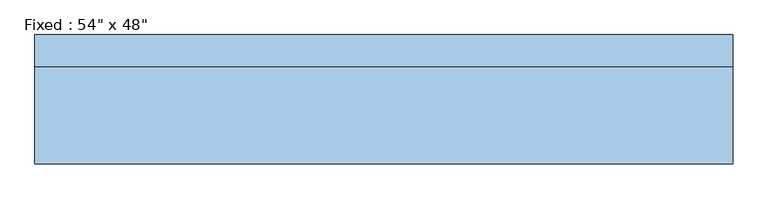
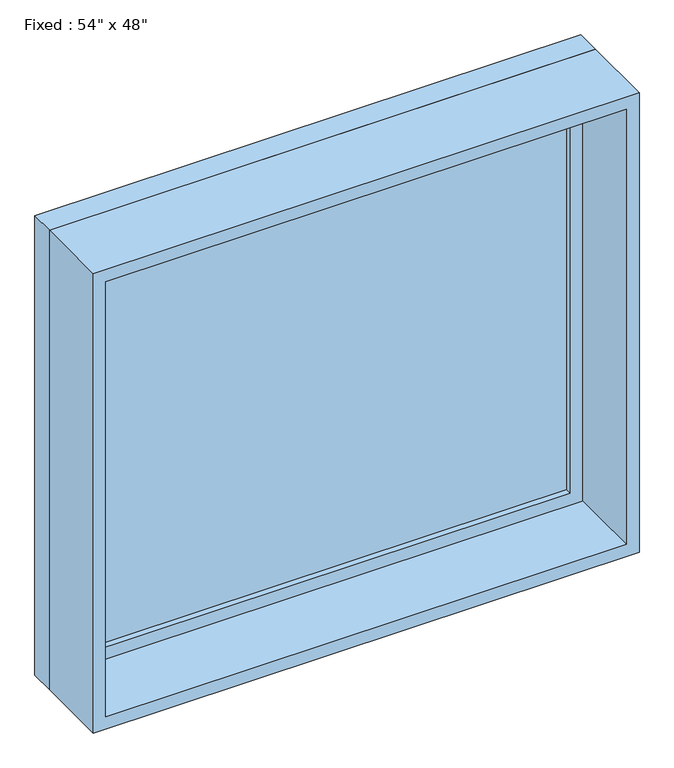
"""IFC4 building model written with IfcOpenShell, lengths in millimetres: window geometry."""

import ifcopenshell
import ifcopenshell.guid

model = None  # the IFC model being written
_history = None  # IfcOwnerHistory: only IFC2X3 demands one
_inside = {}  # id of a spatial element -> (the spatial element, [elements in it])
_under = {}  # id of a project, library or spatial element -> (it, [spatial elements below it])
_declared = {}  # id of a project -> (the project, [libraries it declares])
_typed = {}  # id of a type object -> (the type object, [elements of that type])
_made_of = {}  # id of a material, layer set ... -> (it, [elements and type objects made of it])


def new_model(schema):
    """Start an empty IFC model of exactly this schema.

    Asked for "IFC4X3", IfcOpenShell would pick the latest addendum, in which some entities
    have other attributes; the version numbers below select the first issue.
    IFC2X3 requires an IfcOwnerHistory on every rooted entity: one is made here for all.
    """
    global model, _history
    if schema == "IFC4X3":
        model = ifcopenshell.file(schema_version=(4, 3, 0, 0))
    else:
        model = ifcopenshell.file(schema=schema)
    _inside.clear()
    _under.clear()
    _declared.clear()
    _typed.clear()
    _made_of.clear()
    _history = None
    if model.schema == "IFC2X3":
        org = make("IfcOrganization", Name="unknown")
        user = make(
            "IfcPersonAndOrganization",
            ThePerson=make("IfcPerson", FamilyName="unknown"),
            TheOrganization=org,
        )
        app = make(
            "IfcApplication",
            ApplicationDeveloper=org,
            Version="unknown",
            ApplicationFullName="unknown",
            ApplicationIdentifier="unknown",
        )
        _history = make(
            "IfcOwnerHistory",
            OwningUser=user,
            OwningApplication=app,
            ChangeAction="ADDED",
            CreationDate=0,
        )
    return model


def make(cls, **values):
    """One entity of the class cls with the attributes given. An attribute that is None is left unset."""
    return model.create_entity(
        cls, **{name: value for name, value in values.items() if value is not None}
    )


def rooted(cls, **values):
    """An entity with a GlobalId (a new one), such as an element, a storey or a relation."""
    return make(cls, GlobalId=ifcopenshell.guid.new(), OwnerHistory=_history, **values)


def si_unit(unit_type, name, prefix=None):
    """IfcSIUnit, for example si_unit("LENGTHUNIT", "METRE", prefix="MILLI")."""
    return make("IfcSIUnit", UnitType=unit_type, Prefix=prefix, Name=name)


def assignment(units):
    """IfcUnitAssignment: the units of a project."""
    return None if units is None else make("IfcUnitAssignment", Units=units)


def point(xyz):
    """IfcCartesianPoint."""
    return None if xyz is None else make("IfcCartesianPoint", Coordinates=xyz)


def direction(xyz):
    """IfcDirection."""
    return None if xyz is None else make("IfcDirection", DirectionRatios=xyz)


def frame(location, z_axis=None, x_axis=None):
    """IfcAxis2Placement3D, a coordinate frame: its origin and axes. An axis left out is left unset."""
    return make(
        "IfcAxis2Placement3D",
        Location=point(location),
        Axis=direction(z_axis),
        RefDirection=direction(x_axis),
    )


def origin():
    """The frame at (0, 0, 0) with its axes left unset."""
    return frame((0.0, 0.0, 0.0))


def place(relative_to, where):
    """IfcLocalPlacement: puts the frame where relative to a parent placement (None: the world)."""
    return make(
        "IfcLocalPlacement", PlacementRelTo=relative_to, RelativePlacement=where
    )


def context(
    kind, dimensions, precision=None, world=None, true_north=None, identifier=None
):
    """IfcGeometricRepresentationContext, for example the 3D "Model" context."""
    return make(
        "IfcGeometricRepresentationContext",
        ContextIdentifier=identifier,
        ContextType=kind,
        CoordinateSpaceDimension=dimensions,
        Precision=precision,
        WorldCoordinateSystem=world,
        TrueNorth=true_north,
    )


def project(units=None, contexts=None):
    """IfcProject with its units and contexts."""
    return rooted(
        "IfcProject",
        Name="project",
        RepresentationContexts=contexts,
        UnitsInContext=assignment(units),
    )


def spatial(cls, under=None, at=None, **own):
    """A site, building, storey or space (cls), placed at a placement, below another one or the project."""
    s = rooted(cls, ObjectPlacement=at, **own)
    if under is not None:
        _under.setdefault(under.id(), (under, []))[1].append(s)
    return s


def polyline(points):
    """IfcPolyline through the points."""
    return make("IfcPolyline", Points=[point(p) for p in points])


def outline(outer, holes=None, kind="AREA"):
    """IfcArbitraryClosedProfileDef: a profile drawn as a closed curve; with holes, ...WithVoids."""
    if holes is None:
        return make("IfcArbitraryClosedProfileDef", ProfileType=kind, OuterCurve=outer)
    return make(
        "IfcArbitraryProfileDefWithVoids",
        ProfileType=kind,
        OuterCurve=outer,
        InnerCurves=holes,
    )


def extrude(swept, where, along, depth):
    """IfcExtrudedAreaSolid: the profile swept, set in the frame where, extruded along a direction by depth."""
    return make(
        "IfcExtrudedAreaSolid",
        SweptArea=swept,
        Position=where,
        ExtrudedDirection=direction(along),
        Depth=depth,
    )


def shape(context_of_items, identifier, shape_type, items):
    """IfcShapeRepresentation: the items that make up one representation, for example the "Body"."""
    return make(
        "IfcShapeRepresentation",
        ContextOfItems=context_of_items,
        RepresentationIdentifier=identifier,
        RepresentationType=shape_type,
        Items=items,
    )


def source(mapping_origin, context_of_items, identifier, shape_type, items):
    """IfcRepresentationMap: a shape defined once, which mapped items show again and again."""
    return make(
        "IfcRepresentationMap",
        MappingOrigin=mapping_origin,
        MappedRepresentation=shape(context_of_items, identifier, shape_type, items),
    )


def transform(
    local_origin,
    x_axis=None,
    y_axis=None,
    z_axis=None,
    scale=None,
    scale2=None,
    scale3=None,
    uniform=True,
):
    """IfcCartesianTransformationOperator3D, or its non-uniform kind. x_axis, y_axis, z_axis: its Axis1, 2, 3."""
    if uniform:
        return make(
            "IfcCartesianTransformationOperator3D",
            Axis1=direction(x_axis),
            Axis2=direction(y_axis),
            LocalOrigin=point(local_origin),
            Scale=scale,
            Axis3=direction(z_axis),
        )
    return make(
        "IfcCartesianTransformationOperator3DnonUniform",
        Axis1=direction(x_axis),
        Axis2=direction(y_axis),
        LocalOrigin=point(local_origin),
        Scale=scale,
        Axis3=direction(z_axis),
        Scale2=scale2,
        Scale3=scale3,
    )


def mapped(mapping_source, mapping_target):
    """IfcMappedItem: shows the shape of a source again, moved by a transform."""
    return make(
        "IfcMappedItem", MappingSource=mapping_source, MappingTarget=mapping_target
    )


def made_of(thing, what):
    """Note that an element or type object is made of a material, layer set ...; save() writes the relation."""
    if what is not None:
        _made_of.setdefault(what.id(), (what, []))[1].append(thing)
    return thing


def element(
    cls,
    number,
    at=None,
    inside=None,
    cuts=None,
    type_object=None,
    material=None,
    context=None,
    identifier="Body",
    shape_type=None,
    held_by="IfcProductDefinitionShape",
    body=None,
    shapes=None,
    **own,
):
    """One element of the class cls, such as IfcWall. Its Tag is "e" and its number.

    at: its placement. inside: the storey or other place that contains it. cuts: it is an
    opening in that element (IfcRelVoidsElement). A single representation is given by context,
    identifier, shape_type and body (its items); several are given by shapes. held_by: the class
    of the entity that holds the representations. save() writes the other relations.
    """
    e = rooted(cls, Tag="e%d" % number, ObjectPlacement=at, **own)
    if body is not None:
        shapes = [shape(context, identifier, shape_type, body)]
    if shapes is not None:
        e.Representation = make(held_by, Representations=shapes)
    if inside is not None:
        _inside.setdefault(inside.id(), (inside, []))[1].append(e)
    if cuts is not None:
        rooted(
            "IfcRelVoidsElement", RelatingBuildingElement=cuts, RelatedOpeningElement=e
        )
    if type_object is not None:
        _typed.setdefault(type_object.id(), (type_object, []))[1].append(e)
    return made_of(e, material)


def aggregate(whole, parts):
    """IfcRelAggregates: a whole, such as a stair, and the parts it consists of."""
    return rooted("IfcRelAggregates", RelatingObject=whole, RelatedObjects=parts)


def save(model, path):
    """Write the relations noted so far, then the file.

    IfcRelAggregates (storeys below a building ...), IfcRelContainedInSpatialStructure (elements
    in a storey), IfcRelDefinesByType, IfcRelAssociatesMaterial and IfcRelDeclares: one each for
    every whole, place, type object, material and project.
    """
    for whole, parts in _under.values():
        aggregate(whole, parts)
    for where, things in _inside.values():
        rooted(
            "IfcRelContainedInSpatialStructure",
            RelatedElements=things,
            RelatingStructure=where,
        )
    for kind, things in _typed.values():
        rooted("IfcRelDefinesByType", RelatedObjects=things, RelatingType=kind)
    for what, things in _made_of.values():
        rooted("IfcRelAssociatesMaterial", RelatedObjects=things, RelatingMaterial=what)
    for by, libraries in _declared.values():
        rooted("IfcRelDeclares", RelatingContext=by, RelatedDefinitions=libraries)
    model.write(path)


def window_8bc8f9b7(model_context):
    return source(origin(), model_context, "Body", "SweptSolid", [
        extrude(outline(polyline([(584.2, 79.375), (-660.4, 79.375), (-660.4, 92.075), (584.2, 92.075), (584.2, 79.375)])), frame((0.0, 0.0, 368.3), z_axis=(0.0, 0.0, 1.0), x_axis=(1.0, 0.0, 0.0)), (0.0, 0.0, 1.0), 1092.2),
        extrude(outline(polyline([(1504.95, -704.85), (323.85, -704.85), (323.85, 628.65), (1504.95, 628.65), (1504.95, -704.85)]), holes=[polyline([(1460.5, -660.4), (1460.5, 584.2), (368.3, 584.2), (368.3, -660.4), (1460.5, -660.4)])]), frame((0.0, 63.5, 0.0), z_axis=(0.0, 1.0, 0.0), x_axis=(0.0, 0.0, 1.0)), (0.0, 0.0, 1.0), 44.45),
        extrude(outline(polyline([(1524.0, -723.9), (304.8, -723.9), (304.8, 647.7), (1524.0, 647.7), (1524.0, -723.9)]), holes=[polyline([(1492.25, -692.15), (1492.25, 615.95), (336.55, 615.95), (336.55, -692.15), (1492.25, -692.15)])]), frame((0.0, -127.0, 0.0), z_axis=(0.0, 1.0, 0.0), x_axis=(0.0, 0.0, 1.0)), (0.0, 0.0, 1.0), 190.5),
        extrude(outline(polyline([(1524.0, 647.7), (1524.0, -723.9), (304.8, -723.9), (304.8, 647.7), (1524.0, 647.7)]), holes=[polyline([(1504.95, 628.65), (323.85, 628.65), (323.85, -704.85), (1504.95, -704.85), (1504.95, 628.65)])]), frame((0.0, 63.5, 0.0), z_axis=(0.0, 1.0, 0.0), x_axis=(0.0, 0.0, 1.0)), (0.0, 0.0, 1.0), 63.5),
    ])


if __name__ == "__main__":
    model = new_model("IFC4")
    model_context = context("Model", 3, world=origin())
    ifc_project = project(units=[si_unit("LENGTHUNIT", "METRE", prefix="MILLI")], contexts=[model_context])
    site = spatial("IfcSite", under=ifc_project)
    building = spatial("IfcBuilding", under=site)
    placement = place(None, origin())
    window_shape = window_8bc8f9b7(model_context)
    element("IfcWindow", 1, ObjectType="Fixed : 54\" x 48\"", at=placement, inside=building, context=model_context, shape_type="MappedRepresentation", body=[
        mapped(window_shape, transform((0.0, 0.0, 0.0), x_axis=(1.0, 0.0, 0.0), y_axis=(0.0, 1.0, 0.0), z_axis=(0.0, 0.0, 1.0))),
    ])
    save(model, "model.ifc")

# Revit data of these elements
# Type "Fixed : 54\" x 48\""
#   Type Mark = "12"
#   Assembly Code = "B2020100"
#   Height = 1219.2 mm
#   Default Sill Height = 304.8 mm
#   Width = 1371.6 mm
#   Window Inset = 19.05 mm
#   Glass Pane Material = Glass
#   Sash Material = Sash
#   Wall Closure = (empty or 0)
# Element 1 (IfcWindow, "Fixed : 54\" x 48\"")
#   Materials on its faces: "Sash", "Glass"
# Materials
#   "Glass": class "Glass", colour RGB 0 128 192, transparency 0.75
#   "Sash": class "Wood", colour RGB 224 178 126, transparency 0
